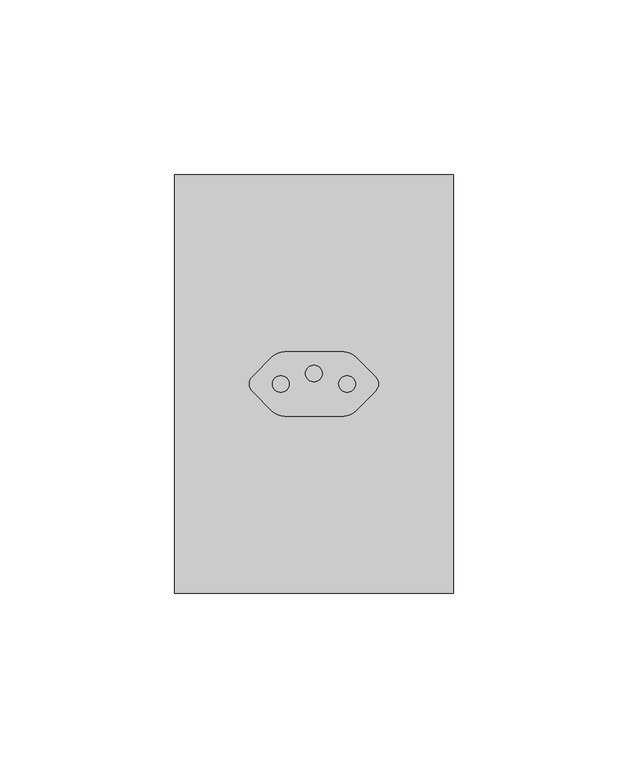
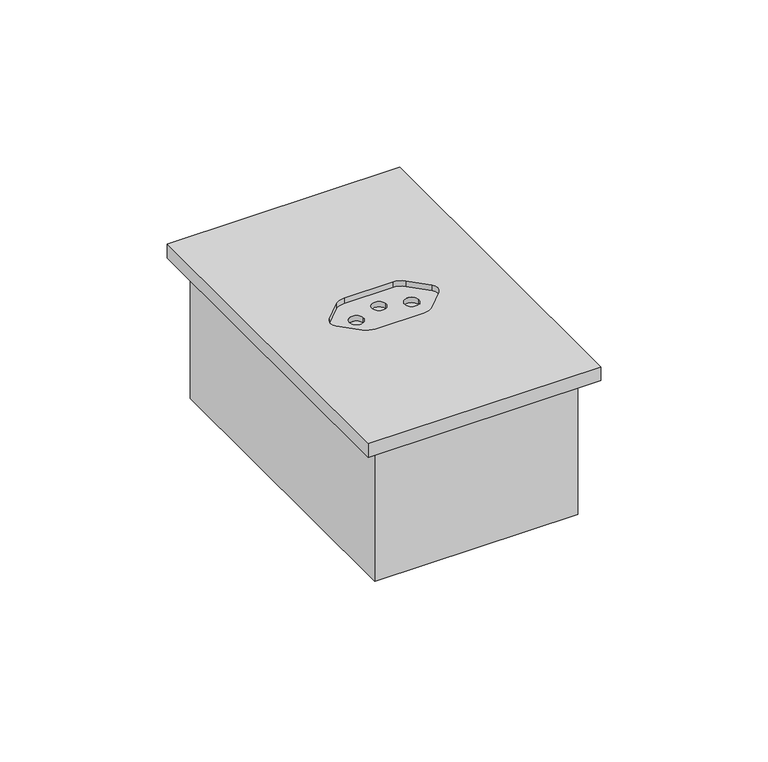
"""IFC4 building model written with IfcOpenShell, lengths in millimetres: proxy geometry, CAIXA VERTICE V7 : Tomada 20A 1s."""

import ifcopenshell
import ifcopenshell.guid

model = None  # the IFC model being written
_history = None  # IfcOwnerHistory: only IFC2X3 demands one
_inside = {}  # id of a spatial element -> (the spatial element, [elements in it])
_under = {}  # id of a project, library or spatial element -> (it, [spatial elements below it])
_declared = {}  # id of a project -> (the project, [libraries it declares])
_typed = {}  # id of a type object -> (the type object, [elements of that type])
_made_of = {}  # id of a material, layer set ... -> (it, [elements and type objects made of it])


def new_model(schema):
    """Start an empty IFC model of exactly this schema.

    Asked for "IFC4X3", IfcOpenShell would pick the latest addendum, in which some entities
    have other attributes; the version numbers below select the first issue.
    IFC2X3 requires an IfcOwnerHistory on every rooted entity: one is made here for all.
    """
    global model, _history
    if schema == "IFC4X3":
        model = ifcopenshell.file(schema_version=(4, 3, 0, 0))
    else:
        model = ifcopenshell.file(schema=schema)
    _inside.clear()
    _under.clear()
    _declared.clear()
    _typed.clear()
    _made_of.clear()
    _history = None
    if model.schema == "IFC2X3":
        org = make("IfcOrganization", Name="unknown")
        user = make(
            "IfcPersonAndOrganization",
            ThePerson=make("IfcPerson", FamilyName="unknown"),
            TheOrganization=org,
        )
        app = make(
            "IfcApplication",
            ApplicationDeveloper=org,
            Version="unknown",
            ApplicationFullName="unknown",
            ApplicationIdentifier="unknown",
        )
        _history = make(
            "IfcOwnerHistory",
            OwningUser=user,
            OwningApplication=app,
            ChangeAction="ADDED",
            CreationDate=0,
        )
    return model


def make(cls, **values):
    """One entity of the class cls with the attributes given. An attribute that is None is left unset."""
    return model.create_entity(
        cls, **{name: value for name, value in values.items() if value is not None}
    )


def rooted(cls, **values):
    """An entity with a GlobalId (a new one), such as an element, a storey or a relation."""
    return make(cls, GlobalId=ifcopenshell.guid.new(), OwnerHistory=_history, **values)


def si_unit(unit_type, name, prefix=None):
    """IfcSIUnit, for example si_unit("LENGTHUNIT", "METRE", prefix="MILLI")."""
    return make("IfcSIUnit", UnitType=unit_type, Prefix=prefix, Name=name)


def assignment(units):
    """IfcUnitAssignment: the units of a project."""
    return None if units is None else make("IfcUnitAssignment", Units=units)


def point(xyz):
    """IfcCartesianPoint."""
    return None if xyz is None else make("IfcCartesianPoint", Coordinates=xyz)


def direction(xyz):
    """IfcDirection."""
    return None if xyz is None else make("IfcDirection", DirectionRatios=xyz)


def frame(location, z_axis=None, x_axis=None):
    """IfcAxis2Placement3D, a coordinate frame: its origin and axes. An axis left out is left unset."""
    return make(
        "IfcAxis2Placement3D",
        Location=point(location),
        Axis=direction(z_axis),
        RefDirection=direction(x_axis),
    )


def origin():
    """The frame at (0, 0, 0) with its axes left unset."""
    return frame((0.0, 0.0, 0.0))


def place(relative_to, where):
    """IfcLocalPlacement: puts the frame where relative to a parent placement (None: the world)."""
    return make(
        "IfcLocalPlacement", PlacementRelTo=relative_to, RelativePlacement=where
    )


def context(
    kind, dimensions, precision=None, world=None, true_north=None, identifier=None
):
    """IfcGeometricRepresentationContext, for example the 3D "Model" context."""
    return make(
        "IfcGeometricRepresentationContext",
        ContextIdentifier=identifier,
        ContextType=kind,
        CoordinateSpaceDimension=dimensions,
        Precision=precision,
        WorldCoordinateSystem=world,
        TrueNorth=true_north,
    )


def project(units=None, contexts=None):
    """IfcProject with its units and contexts."""
    return rooted(
        "IfcProject",
        Name="project",
        RepresentationContexts=contexts,
        UnitsInContext=assignment(units),
    )


def spatial(cls, under=None, at=None, **own):
    """A site, building, storey or space (cls), placed at a placement, below another one or the project."""
    s = rooted(cls, ObjectPlacement=at, **own)
    if under is not None:
        _under.setdefault(under.id(), (under, []))[1].append(s)
    return s


def polyline(points):
    """IfcPolyline through the points."""
    return make("IfcPolyline", Points=[point(p) for p in points])


def circle_curve(where, radius):
    """IfcCircle in the frame where."""
    return make("IfcCircle", Position=where, Radius=radius)


def faces_of(points, faces, orient=None, outer=None):
    """IfcFace entities. A face is a list of loops; a loop is a list of indices into points, from 0.

    orient and outer hold one flag for each loop. By default every Orientation is true, the
    first loop of a face is its IfcFaceOuterBound and the others are IfcFaceBound.
    """
    made = []
    for i, loops in enumerate(faces):
        bounds = []
        for j, loop in enumerate(loops):
            is_outer = j == 0 if outer is None else outer[i][j]
            bounds.append(
                make(
                    "IfcFaceOuterBound" if is_outer else "IfcFaceBound",
                    Bound=make("IfcPolyLoop", Polygon=[points[k] for k in loop]),
                    Orientation=True if orient is None else orient[i][j],
                )
            )
        made.append(make("IfcFace", Bounds=bounds))
    return made


def faceted_brep(points, faces, orient=None, outer=None, voids=None):
    """IfcFacetedBrep: a solid bounded by flat faces; with voids (closed shells), ...WithVoids."""
    shared = [point(p) for p in points]
    hull = make("IfcClosedShell", CfsFaces=faces_of(shared, faces, orient, outer))
    if voids is None:
        return make("IfcFacetedBrep", Outer=hull)
    return make(
        "IfcFacetedBrepWithVoids",
        Outer=hull,
        Voids=[
            make(cls, CfsFaces=faces_of(shared, fs, o, b)) for cls, fs, o, b in voids
        ],
    )


def shape(context_of_items, identifier, shape_type, items):
    """IfcShapeRepresentation: the items that make up one representation, for example the "Body"."""
    return make(
        "IfcShapeRepresentation",
        ContextOfItems=context_of_items,
        RepresentationIdentifier=identifier,
        RepresentationType=shape_type,
        Items=items,
    )


def source(mapping_origin, context_of_items, identifier, shape_type, items):
    """IfcRepresentationMap: a shape defined once, which mapped items show again and again."""
    return make(
        "IfcRepresentationMap",
        MappingOrigin=mapping_origin,
        MappedRepresentation=shape(context_of_items, identifier, shape_type, items),
    )


def transform(
    local_origin,
    x_axis=None,
    y_axis=None,
    z_axis=None,
    scale=None,
    scale2=None,
    scale3=None,
    uniform=True,
):
    """IfcCartesianTransformationOperator3D, or its non-uniform kind. x_axis, y_axis, z_axis: its Axis1, 2, 3."""
    if uniform:
        return make(
            "IfcCartesianTransformationOperator3D",
            Axis1=direction(x_axis),
            Axis2=direction(y_axis),
            LocalOrigin=point(local_origin),
            Scale=scale,
            Axis3=direction(z_axis),
        )
    return make(
        "IfcCartesianTransformationOperator3DnonUniform",
        Axis1=direction(x_axis),
        Axis2=direction(y_axis),
        LocalOrigin=point(local_origin),
        Scale=scale,
        Axis3=direction(z_axis),
        Scale2=scale2,
        Scale3=scale3,
    )


def mapped(mapping_source, mapping_target):
    """IfcMappedItem: shows the shape of a source again, moved by a transform."""
    return make(
        "IfcMappedItem", MappingSource=mapping_source, MappingTarget=mapping_target
    )


def made_of(thing, what):
    """Note that an element or type object is made of a material, layer set ...; save() writes the relation."""
    if what is not None:
        _made_of.setdefault(what.id(), (what, []))[1].append(thing)
    return thing


def element(
    cls,
    number,
    at=None,
    inside=None,
    cuts=None,
    type_object=None,
    material=None,
    context=None,
    identifier="Body",
    shape_type=None,
    held_by="IfcProductDefinitionShape",
    body=None,
    shapes=None,
    **own,
):
    """One element of the class cls, such as IfcWall. Its Tag is "e" and its number.

    at: its placement. inside: the storey or other place that contains it. cuts: it is an
    opening in that element (IfcRelVoidsElement). A single representation is given by context,
    identifier, shape_type and body (its items); several are given by shapes. held_by: the class
    of the entity that holds the representations. save() writes the other relations.
    """
    e = rooted(cls, Tag="e%d" % number, ObjectPlacement=at, **own)
    if body is not None:
        shapes = [shape(context, identifier, shape_type, body)]
    if shapes is not None:
        e.Representation = make(held_by, Representations=shapes)
    if inside is not None:
        _inside.setdefault(inside.id(), (inside, []))[1].append(e)
    if cuts is not None:
        rooted(
            "IfcRelVoidsElement", RelatingBuildingElement=cuts, RelatedOpeningElement=e
        )
    if type_object is not None:
        _typed.setdefault(type_object.id(), (type_object, []))[1].append(e)
    return made_of(e, material)


def aggregate(whole, parts):
    """IfcRelAggregates: a whole, such as a stair, and the parts it consists of."""
    return rooted("IfcRelAggregates", RelatingObject=whole, RelatedObjects=parts)


def save(model, path):
    """Write the relations noted so far, then the file.

    IfcRelAggregates (storeys below a building ...), IfcRelContainedInSpatialStructure (elements
    in a storey), IfcRelDefinesByType, IfcRelAssociatesMaterial and IfcRelDeclares: one each for
    every whole, place, type object, material and project.
    """
    for whole, parts in _under.values():
        aggregate(whole, parts)
    for where, things in _inside.values():
        rooted(
            "IfcRelContainedInSpatialStructure",
            RelatedElements=things,
            RelatingStructure=where,
        )
    for kind, things in _typed.values():
        rooted("IfcRelDefinesByType", RelatedObjects=things, RelatingType=kind)
    for what, things in _made_of.values():
        rooted("IfcRelAssociatesMaterial", RelatedObjects=things, RelatingMaterial=what)
    for by, libraries in _declared.values():
        rooted("IfcRelDeclares", RelatingContext=by, RelatedDefinitions=libraries)
    model.write(path)


def plane_surface(at):
    """IfcPlane: the flat surface through the origin of the frame at, square to its z axis."""
    return make("IfcPlane", Position=at)


def revolved_surface(curve, axis_point, axis_direction):
    """IfcSurfaceOfRevolution: the curve turned about the line through axis_point along axis_direction."""
    return make(
        "IfcSurfaceOfRevolution",
        SweptCurve=make("IfcArbitraryOpenProfileDef", ProfileType="CURVE", Curve=curve),
        AxisPosition=make("IfcAxis1Placement", Location=point(axis_point), Axis=direction(axis_direction)),
    )


def advanced_brep(points, edges, surfaces, faces):
    """IfcAdvancedBrep: a solid bounded by faces that lie on surfaces and meet in shared edges.

    An edge is (start, end): straight between two places in points (the first is 0);
    or (start, end, curve); or (start, end, curve, False) where it runs against its curve.
    A face is (place in surfaces, loops), or (place, loops, False) where it looks against
    its surface's normal. A loop lists edges by number (the first is 1), with a minus sign
    where the edge is run from its end to its start. The first loop is the outer one.
    """
    corners = [point(p) for p in points]
    vertices = [make("IfcVertexPoint", VertexGeometry=c) for c in corners]
    made = []
    for start, end, *more in edges:
        made.append(
            make(
                "IfcEdgeCurve",
                EdgeStart=vertices[start],
                EdgeEnd=vertices[end],
                EdgeGeometry=more[0] if more else make("IfcPolyline", Points=[corners[start], corners[end]]),
                SameSense=more[1] if len(more) > 1 else True,
            )
        )
    hull = []
    for where, loops, *sense in faces:
        bounds = []
        for j, loop in enumerate(loops):
            ring = [make("IfcOrientedEdge", EdgeElement=made[abs(k) - 1], Orientation=k > 0) for k in loop]
            bounds.append(
                make(
                    "IfcFaceOuterBound" if j == 0 else "IfcFaceBound",
                    Bound=make("IfcEdgeLoop", EdgeList=ring),
                    Orientation=True,
                )
            )
        hull.append(make("IfcAdvancedFace", Bounds=bounds, FaceSurface=surfaces[where], SameSense=sense[0] if sense else True))
    return make("IfcAdvancedBrep", Outer=make("IfcClosedShell", CfsFaces=hull))


def electrical_fixtures_6ddb2cd4(model_context):
    return source(origin(), model_context, "Body", "SolidModel", [
        faceted_brep([(33.0, 2147.0, -48.0), (33.0, 2253.0, -48.0), (-33.0, 2253.0, -48.0), (-33.0, 2147.0, -48.0), (35.0, 2255.0, -50.0), (35.0, 2145.0, -50.0), (-35.0, 2145.0, -50.0), (-35.0, 2255.0, -50.0), (-35.0, 2255.0, 0.0), (35.0, 2255.0, 0.0), (-35.0, 2145.0, 0.0), (35.0, 2145.0, 0.0), (33.0, 2253.0, 0.0), (33.0, 2147.0, 0.0), (-33.0, 2147.0, 0.0), (-33.0, 2253.0, 0.0)], [[[0, 1, 2, 3]], [[4, 5, 6, 7]], [[4, 7, 8, 9]], [[8, 7, 6, 10]], [[10, 6, 5, 11]], [[11, 5, 4, 9]], [[9, 8, 10, 11], [12, 13, 14, 15]], [[13, 12, 1, 0]], [[14, 13, 0, 3]], [[15, 14, 3, 2]], [[12, 15, 2, 1]]]),
        advanced_brep(
        [(40.0, 2260.0, 5.0), (-40.0, 2260.0, 5.0), (-40.0, 2140.0, 5.0), (40.0, 2140.0, 5.0), (8.4215729, 2190.75, 5.0), (-8.4215729, 2190.75, 5.0), (-11.9571068, 2192.2144661, 5.0), (-17.6213203, 2197.8786797, 5.0), (-17.6213203, 2202.1213203, 5.0), (-11.9571068, 2207.7855339, 5.0), (-8.4215729, 2209.25, 5.0), (8.4215729, 2209.25, 5.0), (11.9571068, 2207.7855339, 5.0), (17.6213203, 2202.1213203, 5.0), (17.6213203, 2197.8786797, 5.0), (11.9571068, 2192.2144661, 5.0), (-40.0, 2260.0, 0.0), (40.0, 2260.0, 0.0), (40.0, 2140.0, 0.0), (-40.0, 2140.0, 0.0), (8.4215729, 2190.75, 3.0), (11.9571068, 2192.2144661, 3.0), (17.6213203, 2197.8786797, 3.0), (17.6213203, 2202.1213203, 3.0), (11.9571068, 2207.7855339, 3.0), (8.4215729, 2209.25, 3.0), (-8.4215729, 2209.25, 3.0), (-11.9571068, 2207.7855339, 3.0), (-17.6213203, 2202.1213203, 3.0), (-17.6213203, 2197.8786797, 3.0), (-11.9571068, 2192.2144661, 3.0), (-8.4215729, 2190.75, 3.0), (-7.1, 2200.0, 3.0), (-11.9, 2200.0, 3.0), (11.9, 2200.0, 3.0), (7.1, 2200.0, 3.0), (2.4, 2203.0, 3.0), (-2.4, 2203.0, 3.0), (-11.9, 2200.0, 1.0), (-7.1, 2200.0, 1.0), (7.1, 2200.0, 1.0), (11.9, 2200.0, 1.0), (-2.4, 2203.0, 1.0), (2.4, 2203.0, 1.0)],
        [
            (0, 1),
            (1, 2),
            (2, 3),
            (3, 0),
            (4, 5),
            (5, 6, circle_curve(frame((-8.4215729, 2195.75, 5.0), z_axis=(0.0, 0.0, -1.0), x_axis=(-1.0, 0.0, 0.0)), 5.0)),
            (6, 7),
            (7, 8, circle_curve(frame((-15.5, 2200.0, 5.0), z_axis=(0.0, 0.0, -1.0), x_axis=(-1.0, 0.0, 0.0)), 3.0)),
            (8, 9),
            (9, 10, circle_curve(frame((-8.4215729, 2204.25, 5.0), z_axis=(0.0, 0.0, -1.0), x_axis=(-1.0, 0.0, 0.0)), 5.0)),
            (10, 11),
            (11, 12, circle_curve(frame((8.4215729, 2204.25, 5.0), z_axis=(0.0, 0.0, -1.0), x_axis=(-1.0, 0.0, 0.0)), 5.0)),
            (12, 13),
            (13, 14, circle_curve(frame((15.5, 2200.0, 5.0), z_axis=(0.0, 0.0, -1.0), x_axis=(-1.0, 0.0, 0.0)), 3.0)),
            (14, 15),
            (15, 4, circle_curve(frame((8.4215729, 2195.75, 5.0), z_axis=(0.0, 0.0, -1.0), x_axis=(-1.0, 0.0, 0.0)), 5.0)),
            (16, 17),
            (17, 18),
            (18, 19),
            (19, 16),
            (0, 17),
            (16, 1),
            (19, 2),
            (18, 3),
            (20, 21, circle_curve(frame((8.4215729, 2195.75, 3.0), z_axis=(0.0, 0.0, 1.0), x_axis=(-1.0, 0.0, 0.0)), 5.0)),
            (21, 22),
            (22, 23, circle_curve(frame((15.5, 2200.0, 3.0), z_axis=(0.0, 0.0, 1.0), x_axis=(-1.0, 0.0, 0.0)), 3.0)),
            (23, 24),
            (24, 25, circle_curve(frame((8.4215729, 2204.25, 3.0), z_axis=(0.0, 0.0, 1.0), x_axis=(-1.0, 0.0, 0.0)), 5.0)),
            (25, 26),
            (26, 27, circle_curve(frame((-8.4215729, 2204.25, 3.0), z_axis=(0.0, 0.0, 1.0), x_axis=(-1.0, 0.0, 0.0)), 5.0)),
            (27, 28),
            (28, 29, circle_curve(frame((-15.5, 2200.0, 3.0), z_axis=(0.0, 0.0, 1.0), x_axis=(-1.0, 0.0, 0.0)), 3.0)),
            (29, 30),
            (30, 31, circle_curve(frame((-8.4215729, 2195.75, 3.0), z_axis=(0.0, 0.0, 1.0), x_axis=(-1.0, 0.0, 0.0)), 5.0)),
            (31, 20),
            (32, 33, circle_curve(frame((-9.5, 2200.0, 3.0), z_axis=(0.0, 0.0, -1.0), x_axis=(1.0, 2.301812013077709e-12, 0.0)), 2.4)),
            (33, 32, circle_curve(frame((-9.5, 2200.0, 3.0), z_axis=(0.0, 0.0, -1.0), x_axis=(1.0, 2.301812013077709e-12, 0.0)), 2.4)),
            (34, 35, circle_curve(frame((9.5, 2200.0, 3.0), z_axis=(0.0, 0.0, -1.0), x_axis=(1.0, 2.301812013077709e-12, 0.0)), 2.4)),
            (35, 34, circle_curve(frame((9.5, 2200.0, 3.0), z_axis=(0.0, 0.0, -1.0), x_axis=(1.0, 2.301812013077709e-12, 0.0)), 2.4)),
            (36, 37, circle_curve(frame((0.0, 2203.0, 3.0), z_axis=(0.0, 0.0, -1.0), x_axis=(1.0, 2.301812013077709e-12, 0.0)), 2.4)),
            (37, 36, circle_curve(frame((0.0, 2203.0, 3.0), z_axis=(0.0, 0.0, -1.0), x_axis=(1.0, 2.301812013077709e-12, 0.0)), 2.4)),
            (31, 5),
            (4, 20),
            (30, 6),
            (29, 7),
            (28, 8),
            (27, 9),
            (26, 10),
            (25, 11),
            (24, 12),
            (23, 13),
            (22, 14),
            (21, 15),
            (38, 39, circle_curve(frame((-9.5, 2200.0, 1.0), z_axis=(0.0, 0.0, 1.0), x_axis=(1.0, 2.301812013077709e-12, 0.0)), 2.4)),
            (39, 38, circle_curve(frame((-9.5, 2200.0, 1.0), z_axis=(0.0, 0.0, 1.0), x_axis=(1.0, 2.301812013077709e-12, 0.0)), 2.4)),
            (40, 41, circle_curve(frame((9.5, 2200.0, 1.0), z_axis=(0.0, 0.0, 1.0), x_axis=(1.0, 2.301812013077709e-12, 0.0)), 2.4)),
            (41, 40, circle_curve(frame((9.5, 2200.0, 1.0), z_axis=(0.0, 0.0, 1.0), x_axis=(1.0, 2.301812013077709e-12, 0.0)), 2.4)),
            (42, 43, circle_curve(frame((0.0, 2203.0, 1.0), z_axis=(0.0, 0.0, 1.0), x_axis=(1.0, 2.301812013077709e-12, 0.0)), 2.4)),
            (43, 42, circle_curve(frame((0.0, 2203.0, 1.0), z_axis=(0.0, 0.0, 1.0), x_axis=(1.0, 2.301812013077709e-12, 0.0)), 2.4)),
            (32, 39),
            (38, 33),
            (34, 41),
            (40, 35),
            (36, 43),
            (42, 37),
        ],
        [
            plane_surface(frame((-60.0, 2260.0, 5.0), z_axis=(0.0, 0.0, 1.0), x_axis=(-1.0, 0.0, 0.0))),
            plane_surface(frame((-60.0, 2260.0, 0.0), z_axis=(0.0, 0.0, -1.0), x_axis=(1.0, 0.0, 0.0))),
            plane_surface(frame((40.0, 2260.0, 5.0), z_axis=(0.0, 1.0, 0.0), x_axis=(0.0, 0.0, -1.0))),
            plane_surface(frame((-40.0, 2260.0, 5.0), z_axis=(-1.0, 0.0, 0.0), x_axis=(0.0, 0.0, -1.0))),
            plane_surface(frame((-40.0, 2140.0, 5.0), z_axis=(0.0, -1.0, 0.0), x_axis=(0.0, 0.0, -1.0))),
            plane_surface(frame((40.0, 2140.0, 5.0), z_axis=(1.0, 0.0, 0.0), x_axis=(0.0, 0.0, -1.0))),
            plane_surface(frame((3.4215729, 2195.75, 3.0), z_axis=(0.0, 0.0, 1.0), x_axis=(0.0, 1.0, 0.0))),
            plane_surface(frame((-8.4215729, 2190.75, 5.0), z_axis=(0.0, 1.0, 0.0), x_axis=(0.0, 0.0, -1.0))),
            revolved_surface(polyline([(-13.4215729, 2195.75, 5.0), (-13.4215729, 2195.75, 3.0)]), (-8.4215729, 2195.75, 3.0), (0.0, 0.0, 1.0)),
            plane_surface(frame((-17.6213203, 2197.8786797, 5.0), z_axis=(0.7071067811865045, 0.7071067811865905, 0.0), x_axis=(0.0, 0.0, -1.0))),
            revolved_surface(polyline([(-18.5, 2200.0, 5.0), (-18.5, 2200.0, 3.0)]), (-15.5, 2200.0, 3.0), (0.0, 0.0, 1.0)),
            plane_surface(frame((-11.9571068, 2207.7855339, 5.0), z_axis=(0.7071067811865515, -0.7071067811865437, 0.0), x_axis=(0.0, 0.0, -1.0))),
            revolved_surface(polyline([(-13.4215729, 2204.25, 5.0), (-13.4215729, 2204.25, 3.0)]), (-8.4215729, 2204.25, 3.0), (0.0, 0.0, 1.0)),
            plane_surface(frame((8.4215729, 2209.25, 5.0), z_axis=(0.0, -1.0, 0.0), x_axis=(0.0, 0.0, -1.0))),
            revolved_surface(polyline([(3.4215728999999993, 2204.25, 5.0), (3.4215728999999993, 2204.25, 3.0)]), (8.4215729, 2204.25, 3.0), (0.0, 0.0, 1.0)),
            plane_surface(frame((17.6213203, 2202.1213203, 5.0), z_axis=(-0.7071067811865307, -0.7071067811865643, 0.0), x_axis=(0.0, 0.0, -1.0))),
            revolved_surface(polyline([(12.5, 2200.0, 5.0), (12.5, 2200.0, 3.0)]), (15.5, 2200.0, 3.0), (0.0, 0.0, 1.0)),
            plane_surface(frame((11.9571068, 2192.2144661, 5.0), z_axis=(-0.7071067811865893, 0.7071067811865058, 0.0), x_axis=(0.0, 0.0, -1.0))),
            revolved_surface(polyline([(3.4215728999999993, 2195.75, 5.0), (3.4215728999999993, 2195.75, 3.0)]), (8.4215729, 2195.75, 3.0), (0.0, 0.0, 1.0)),
            plane_surface(frame((-7.1, 2200.0, 1.0), z_axis=(0.0, 0.0, 1.0), x_axis=(2.301812013077709e-12, -1.0, 0.0))),
            revolved_surface(polyline([(-7.1, 2200.0000000000055, 3.0), (-7.1, 2200.0000000000055, 1.0)]), (-9.5, 2200.0, 1.0), (0.0, 0.0, 1.0)),
            revolved_surface(polyline([(11.9, 2200.0000000000055, 3.0), (11.9, 2200.0000000000055, 1.0)]), (9.5, 2200.0, 5.0), (0.0, 0.0, 1.0)),
            revolved_surface(polyline([(2.4, 2203.0000000000055, 3.0), (2.4, 2203.0000000000055, 1.0)]), (0.0, 2203.0, 5.0), (0.0, 0.0, 1.0)),
        ],
        [
            (0, [[1, 2, 3, 4], [5, 6, 7, 8, 9, 10, 11, 12, 13, 14, 15, 16]]),
            (1, [[17, 18, 19, 20]]),
            (2, [[-1, 21, -17, 22]]),
            (3, [[-2, -22, -20, 23]]),
            (4, [[-3, -23, -19, 24]]),
            (5, [[-4, -24, -18, -21]]),
            (6, [[25, 26, 27, 28, 29, 30, 31, 32, 33, 34, 35, 36], [37, 38], [39, 40], [41, 42]]),
            (7, [[-36, 43, -5, 44]]),
            (8, [[-35, 45, -6, -43]]),
            (9, [[-34, 46, -7, -45]]),
            (10, [[-33, 47, -8, -46]]),
            (11, [[-32, 48, -9, -47]]),
            (12, [[-31, 49, -10, -48]]),
            (13, [[-30, 50, -11, -49]]),
            (14, [[-29, 51, -12, -50]]),
            (15, [[-28, 52, -13, -51]]),
            (16, [[-27, 53, -14, -52]]),
            (17, [[-26, 54, -15, -53]]),
            (18, [[-25, -44, -16, -54]]),
            (19, [[55, 56]]),
            (19, [[57, 58]]),
            (19, [[59, 60]]),
            (20, [[-37, 61, -55, 62]]),
            (20, [[-38, -62, -56, -61]]),
            (21, [[-39, 63, -57, 64]]),
            (21, [[-40, -64, -58, -63]]),
            (22, [[-41, 65, -59, 66]]),
            (22, [[-42, -66, -60, -65]]),
        ],
    ),
    ])


if __name__ == "__main__":
    model = new_model("IFC4")
    model_context = context("Model", 3, world=origin())
    ifc_project = project(units=[si_unit("LENGTHUNIT", "METRE", prefix="MILLI")], contexts=[model_context])
    site = spatial("IfcSite", under=ifc_project)
    building = spatial("IfcBuilding", under=site)
    placement = place(None, origin())
    electrical_fixtures_shape = electrical_fixtures_6ddb2cd4(model_context)
    element("IfcBuildingElementProxy", 1, Name="CAIXA VERTICE V7 : Tomada 20A 1s", ObjectType="CAIXA VERTICE V7 : Tomada 20A 1s", at=placement, inside=building, context=model_context, shape_type="MappedRepresentation", body=[
        mapped(electrical_fixtures_shape, transform((0.0, 0.0, 0.0), x_axis=(1.0, 0.0, 0.0), y_axis=(0.0, 1.0, 0.0), z_axis=(0.0, 0.0, 1.0))),
    ])
    save(model, "model.ifc")

# Revit data of these elements
# Type "CAIXA VERTICE V7 : Tomada 20A 1s"
#   URL = "www.facebook.com/verticetreinamentos"
#   SEÇÃO [instance default] = ""
#   Rotação [instance default] = 0.00°
#   LARGURA DA TAMPA = 0.08 m
#   BORDA = 0.01 m
#   ALTURA DE INSTALAÇÃO [instance default] = 1.10 m
#   Distância Anotação [instance default] = 0.0015 m
#   ALTURA DA TAMPA = 0.12 m
#   Vertical [instance default] = yes
#   VER SEÇÃO [instance default] = no
#   SHADE ESQ [instance default] = no
#   SHADE DIR [instance default] = yes
#   HORIZONTAL [instance default] = no
#   ANDAR COM A LEGENDA [instance default] = 0
#   Material Tampa [instance default] = Plástico, branco opaco
#   Caixa = element 1798517
#   Anotação = element 1798531
#   Default Elevation = 0
# Element 1 (IfcBuildingElementProxy, "CAIXA VERTICE V7 : Tomada 20A 1s")
#   ALTURA DE INSTALAÇÃO = 2.20 m
#   SHADE ESQ = yes
#   Materials on its faces: "Plástico, branco opaco"
# Materials
#   "Plástico, branco opaco": class "Plástico", colour RGB 120 120 120, transparency 0, Description = "Plastic, generic, opaque white", Cost = 0
